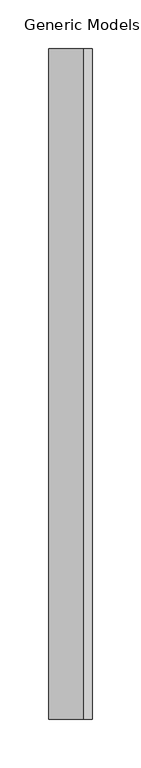
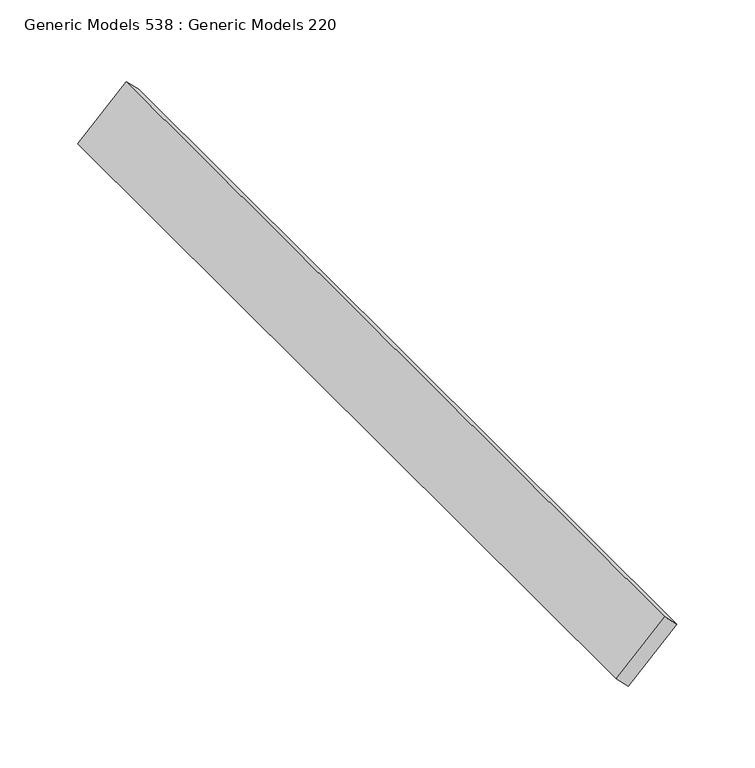
"""IFC4 building model written with IfcOpenShell, lengths in millimetres: proxy geometry, Generic Models 538 : Generic Models 220."""

from ifc_helpers import new_model, si_unit, frame, origin, place, context, project, spatial, polyline, outline, extrude, source, transform, mapped, element, save


def generic_models_538_generic_models_220_1ceccaf3(model_context):
    return source(origin(), model_context, "Body", "SweptSolid", [
        extrude(outline(polyline([(0.0, -12.7000001), (0.0, 0.0), (690.8142348, 0.0), (690.8142348, -12.7000001), (0.0, -12.7000001)])), frame((7841.3059863, 4539.4872686, 125065.1399101), z_axis=(0.7071067811868034, 0.0, 0.7071067811862918), x_axis=(0.0, -1.0, 0.0)), (0.0, 0.0, 1.0), 50.8),
    ])


if __name__ == "__main__":
    model = new_model("IFC4")
    model_context = context("Model", 3, world=origin())
    ifc_project = project(units=[si_unit("LENGTHUNIT", "METRE", prefix="MILLI")], contexts=[model_context])
    site = spatial("IfcSite", under=ifc_project)
    building = spatial("IfcBuilding", under=site)
    placement = place(None, origin())
    generic_models_538_generic_models_220_shape = generic_models_538_generic_models_220_1ceccaf3(model_context)
    element("IfcBuildingElementProxy", 1, Name="Generic Models 538 : Generic Models 220", ObjectType="Generic Models 538 : Generic Models 220", at=placement, inside=building, context=model_context, shape_type="MappedRepresentation", body=[
        mapped(generic_models_538_generic_models_220_shape, transform((0.0, 0.0, 0.0), x_axis=(1.0, 0.0, 0.0), y_axis=(0.0, 1.0, 0.0), z_axis=(0.0, 0.0, 1.0))),
    ])
    save(model, "model.ifc")

# Revit data of these elements
# Element 1 (IfcBuildingElementProxy, "Generic Models 538 : Generic Models 220")
#   Materials on its faces: "_WOOD TONE ALUMINUM EXTRUSION SLAT BY KNOTWOOD"
# Materials
#   "_WOOD TONE ALUMINUM EXTRUSION SLAT BY KNOTWOOD": class "Generic", colour RGB 177 130 114, transparency 0, Cost = 0
